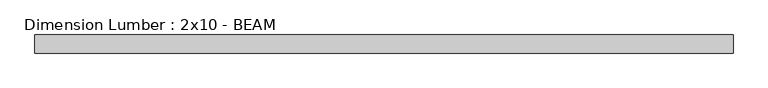
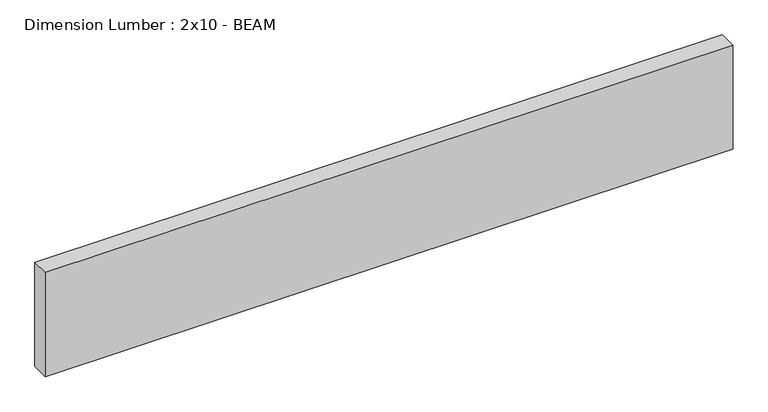
"""IFC4 building model written with IfcOpenShell, lengths in millimetres: beam geometry, Dimension Lumber : 2x10 - BEAM."""

from ifc_helpers import new_model, si_unit, frame, origin, place, context, project, spatial, polyline, outline, extrude, source, transform, mapped, element, save


def dimension_lumber_2x10_beam_ba79c698(model_context):
    return source(origin(), model_context, "Body", "SweptSolid", [
        extrude(outline(polyline([(733.425, 19.05), (733.425, -19.05), (-733.425, -19.05), (-733.425, 19.05), (733.425, 19.05)])), frame((0.0, 0.0, -117.475), z_axis=(0.0, 0.0, 1.0), x_axis=(1.0, 0.0, 0.0)), (0.0, 0.0, 1.0), 234.95),
    ])


if __name__ == "__main__":
    model = new_model("IFC4")
    model_context = context("Model", 3, world=origin())
    ifc_project = project(units=[si_unit("LENGTHUNIT", "METRE", prefix="MILLI")], contexts=[model_context])
    site = spatial("IfcSite", under=ifc_project)
    building = spatial("IfcBuilding", under=site)
    placement = place(None, origin())
    dimension_lumber_2x10_beam_shape = dimension_lumber_2x10_beam_ba79c698(model_context)
    element("IfcBeam", 1, ObjectType="Dimension Lumber : 2x10 - BEAM", at=placement, inside=building, context=model_context, shape_type="MappedRepresentation", body=[
        mapped(dimension_lumber_2x10_beam_shape, transform((0.0, 0.0, 0.0), x_axis=(1.0, 0.0, 0.0), y_axis=(0.0, 1.0, 0.0), z_axis=(0.0, 0.0, 1.0))),
    ])
    save(model, "model.ifc")

# Revit data of these elements
# Type "Dimension Lumber : 2x10 - BEAM"
#   Assembly Code = "B10"
#   A = 0.0755556 SF
#   Length [instance default] = 5' - 0"
#   b = 0' - 1 1/2"
#   d = 0' - 9 1/4"
#   Structural Material = (3) SISTERED 2X10s AT BEAM
# Element 1 (IfcBeam, "Dimension Lumber : 2x10 - BEAM")
#   Materials on its faces: "(3) SISTERED 2X10s AT BEAM"
# Materials
#   "(3) SISTERED 2X10s AT BEAM": class "Wood", colour RGB 234 198 147, transparency 0, Description = "Pinus Echinata", Cost = 0
